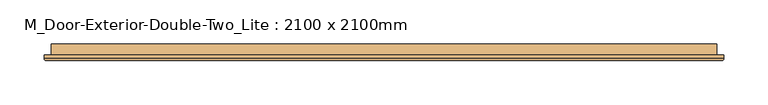
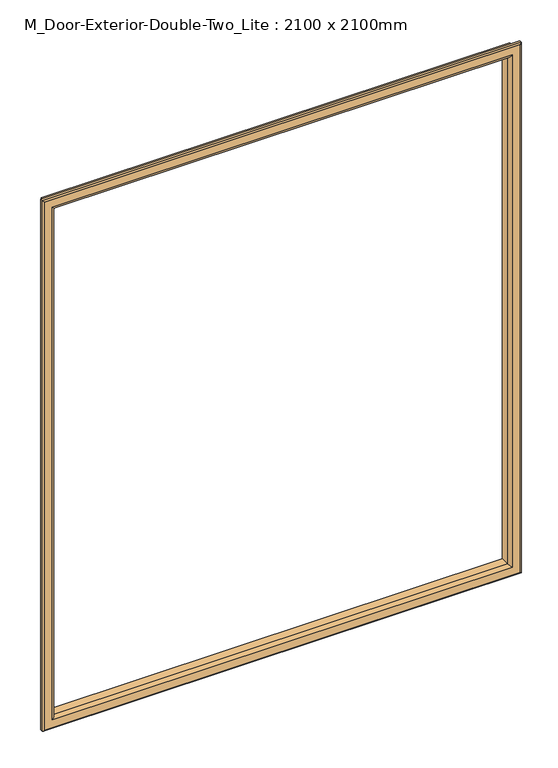
"""IFC4 building model written with IfcOpenShell, lengths in millimetres: door geometry, M_Door-Exterior-Double-Two_Lite : 2100 x 2100mm."""

from ifc_helpers import new_model, si_unit, frame, origin, place, context, project, spatial, ellipse_curve, source, transform, mapped, element, save
from ifc_brep_helpers import plane_surface, cylinder_surface, advanced_brep


def m_door_exterior_double_two_lite_2100_x_2100mm_02d4f706(model_context):
    return source(origin(), model_context, "Body", "AdvancedBrep", [
        advanced_brep(
        [(-900.0, 11.35, 1100.0), (-900.0, -1.15, 1100.0), (-900.0, -1.15, 1980.0), (-900.0, 11.35, 1980.0), (-888.0, -2.15, 1112.0), (-888.0, 11.35, 1112.0), (-888.0, 11.35, 1968.0), (-888.0, -2.15, 1968.0), (-893.0, -7.15, 1107.0), (-893.0, -7.15, 1973.0), (-908.0, -5.15, 1092.0), (-906.0, -7.15, 1094.0), (-906.0, -7.15, 1986.0), (-908.0, -5.15, 1988.0), (-908.0, -1.15, 1092.0), (-908.0, -1.15, 1988.0), (-150.0, -1.15, 1980.0), (-150.0, 11.35, 1980.0), (-162.0, 11.35, 1968.0), (-162.0, -2.15, 1968.0), (-157.0, -7.15, 1973.0), (-144.0, -7.15, 1986.0), (-142.0, -5.15, 1988.0), (-142.0, -1.15, 1988.0), (-150.0, -1.15, 1100.0), (-150.0, 11.35, 1100.0), (-162.0, 11.35, 1112.0), (-162.0, -2.15, 1112.0), (-157.0, -7.15, 1107.0), (-144.0, -7.15, 1094.0), (-142.0, -5.15, 1092.0), (-142.0, -1.15, 1092.0)],
        [
            (0, 1),
            (1, 2),
            (2, 3),
            (3, 0),
            (4, 5),
            (5, 6),
            (6, 7),
            (7, 4),
            (8, 4, ellipse_curve(frame((-893.0, -2.15, 1107.0), z_axis=(-0.7071067811865475, 0.0, 0.7071067811865475), x_axis=(-0.7071067811865474, 0.0, -0.7071067811865476)), 7.0710678, 5.0)),
            (7, 9, ellipse_curve(frame((-893.0, -2.15, 1973.0), z_axis=(-0.7071067811865475, 0.0, -0.7071067811865475), x_axis=(0.7071067811865474, 0.0, -0.7071067811865476)), 7.0710678, 5.0)),
            (9, 8),
            (10, 11, ellipse_curve(frame((-906.0, -5.15, 1094.0), z_axis=(-0.7071067811865475, 0.0, 0.7071067811865475), x_axis=(-0.7071067811865474, 0.0, -0.7071067811865476)), 2.8284271, 2.0)),
            (11, 12),
            (12, 13, ellipse_curve(frame((-906.0, -5.15, 1986.0), z_axis=(-0.7071067811865475, 0.0, -0.7071067811865475), x_axis=(0.7071067811865474, 0.0, -0.7071067811865476)), 2.8284271, 2.0)),
            (13, 10),
            (14, 10),
            (13, 15),
            (15, 14),
            (2, 16),
            (16, 17),
            (17, 3),
            (6, 18),
            (18, 19),
            (19, 7),
            (19, 20, ellipse_curve(frame((-157.0, -2.15, 1973.0), z_axis=(-0.7071067811865475, 0.0, 0.7071067811865475), x_axis=(-0.7071067811865476, 0.0, -0.7071067811865474)), 7.0710678, 5.0)),
            (20, 9),
            (12, 21),
            (21, 22, ellipse_curve(frame((-144.0, -5.15, 1986.0), z_axis=(-0.7071067811865475, 0.0, 0.7071067811865475), x_axis=(-0.7071067811865476, 0.0, -0.7071067811865474)), 2.8284271, 2.0)),
            (22, 13),
            (22, 23),
            (23, 15),
            (16, 24),
            (24, 25),
            (25, 17),
            (18, 26),
            (26, 27),
            (27, 19),
            (27, 28, ellipse_curve(frame((-157.0, -2.15, 1107.0), z_axis=(0.7071067811865475, 0.0, 0.7071067811865475), x_axis=(-0.7071067811865474, 0.0, 0.7071067811865476)), 7.0710678, 5.0)),
            (28, 20),
            (21, 29),
            (29, 30, ellipse_curve(frame((-144.0, -5.15, 1094.0), z_axis=(0.7071067811865475, 0.0, 0.7071067811865475), x_axis=(-0.7071067811865474, 0.0, 0.7071067811865476)), 2.8284271, 2.0)),
            (30, 22),
            (30, 31),
            (31, 23),
            (31, 14),
            (1, 24),
            (0, 25),
            (5, 26),
            (4, 27),
            (8, 28),
            (11, 29),
            (10, 30),
        ],
        [
            plane_surface(frame((-900.0, -1.15, 1100.0), z_axis=(-1.0, 0.0, 0.0), x_axis=(0.0, 0.0, 1.0))),
            plane_surface(frame((-888.0, 11.35, 1112.0), z_axis=(1.0, 0.0, 0.0), x_axis=(0.0, 0.0, 1.0))),
            cylinder_surface(frame((-893.0, -2.15, 1100.0), z_axis=(0.0, 0.0, -1.0), x_axis=(-1.0, 0.0, 0.0)), 5.0),
            cylinder_surface(frame((-906.0, -5.15, 1100.0), z_axis=(0.0, 0.0, -1.0), x_axis=(-1.0, 0.0, 0.0)), 2.0),
            plane_surface(frame((-908.0, -5.15, 1092.0), z_axis=(-1.0, 0.0, 0.0), x_axis=(0.0, 0.0, 1.0))),
            plane_surface(frame((-900.0, -1.15, 1980.0), z_axis=(0.0, 0.0, 1.0), x_axis=(1.0, 0.0, 0.0))),
            plane_surface(frame((-888.0, 11.35, 1968.0), z_axis=(0.0, 0.0, -1.0), x_axis=(1.0, 0.0, 0.0))),
            cylinder_surface(frame((-900.0, -2.15, 1973.0), z_axis=(-1.0, 0.0, 0.0), x_axis=(0.0, 0.0, 1.0)), 5.0),
            cylinder_surface(frame((-900.0, -5.15, 1986.0), z_axis=(-1.0, 0.0, 0.0), x_axis=(0.0, 0.0, 1.0)), 2.0),
            plane_surface(frame((-908.0, -5.15, 1988.0), z_axis=(0.0, 0.0, 1.0), x_axis=(1.0, 0.0, 0.0))),
            plane_surface(frame((-150.0, -1.15, 1980.0), z_axis=(1.0, 0.0, 0.0), x_axis=(0.0, 0.0, -1.0))),
            plane_surface(frame((-162.0, 11.35, 1968.0), z_axis=(-1.0, 0.0, 0.0), x_axis=(0.0, 0.0, -1.0))),
            cylinder_surface(frame((-157.0, -2.15, 1980.0), z_axis=(0.0, 0.0, 1.0), x_axis=(1.0, 0.0, 0.0)), 5.0),
            cylinder_surface(frame((-144.0, -5.15, 1980.0), z_axis=(0.0, 0.0, 1.0), x_axis=(1.0, 0.0, 0.0)), 2.0),
            plane_surface(frame((-142.0, -5.15, 1988.0), z_axis=(1.0, 0.0, 0.0), x_axis=(0.0, 0.0, -1.0))),
            plane_surface(frame((-142.0, -1.15, 1092.0), z_axis=(0.0, 1.0, 0.0), x_axis=(-1.0, 0.0, 0.0))),
            plane_surface(frame((-150.0, -1.15, 1100.0), z_axis=(0.0, 0.0, -1.0), x_axis=(-1.0, 0.0, 0.0))),
            plane_surface(frame((-150.0, 11.35, 1100.0), z_axis=(0.0, 1.0, 0.0), x_axis=(-1.0, 0.0, 0.0))),
            plane_surface(frame((-162.0, 11.35, 1112.0), z_axis=(0.0, 0.0, 1.0), x_axis=(-1.0, 0.0, 0.0))),
            cylinder_surface(frame((-150.0, -2.15, 1107.0), z_axis=(1.0, 0.0, 0.0), x_axis=(0.0, 0.0, -1.0)), 5.0),
            plane_surface(frame((-157.0, -7.15, 1107.0), z_axis=(0.0, -1.0, 0.0), x_axis=(-1.0, 0.0, 0.0))),
            cylinder_surface(frame((-150.0, -5.15, 1094.0), z_axis=(1.0, 0.0, 0.0), x_axis=(0.0, 0.0, -1.0)), 2.0),
            plane_surface(frame((-142.0, -5.15, 1092.0), z_axis=(0.0, 0.0, -1.0), x_axis=(-1.0, 0.0, 0.0))),
        ],
        [
            (0, [[1, 2, 3, 4]]),
            (1, [[5, 6, 7, 8]]),
            (2, [[9, -8, 10, 11]]),
            (3, [[12, 13, 14, 15]]),
            (4, [[16, -15, 17, 18]]),
            (5, [[-3, 19, 20, 21]]),
            (6, [[-7, 22, 23, 24]]),
            (7, [[-10, -24, 25, 26]]),
            (8, [[-14, 27, 28, 29]]),
            (9, [[-17, -29, 30, 31]]),
            (10, [[-20, 32, 33, 34]]),
            (11, [[-23, 35, 36, 37]]),
            (12, [[-25, -37, 38, 39]]),
            (13, [[-28, 40, 41, 42]]),
            (14, [[-30, -42, 43, 44]]),
            (15, [[-31, -44, 45, -18], [46, -32, -19, -2]]),
            (16, [[-33, -46, -1, 47]]),
            (17, [[-21, -34, -47, -4], [48, -35, -22, -6]]),
            (18, [[-36, -48, -5, 49]]),
            (19, [[-38, -49, -9, 50]]),
            (20, [[51, -40, -27, -13], [-26, -39, -50, -11]]),
            (21, [[-41, -51, -12, 52]]),
            (22, [[-43, -52, -16, -45]]),
        ],
    ),
    ])


if __name__ == "__main__":
    model = new_model("IFC4")
    model_context = context("Model", 3, world=origin())
    ifc_project = project(units=[si_unit("LENGTHUNIT", "METRE", prefix="MILLI")], contexts=[model_context])
    site = spatial("IfcSite", under=ifc_project)
    building = spatial("IfcBuilding", under=site)
    placement = place(None, origin())
    m_door_exterior_double_two_lite_2100_x_2100mm_shape = m_door_exterior_double_two_lite_2100_x_2100mm_02d4f706(model_context)
    element("IfcDoor", 1, ObjectType="M_Door-Exterior-Double-Two_Lite : 2100 x 2100mm", at=placement, inside=building, context=model_context, shape_type="MappedRepresentation", body=[
        mapped(m_door_exterior_double_two_lite_2100_x_2100mm_shape, transform((0.0, 0.0, 0.0), x_axis=(1.0, 0.0, 0.0), y_axis=(0.0, 1.0, 0.0), z_axis=(0.0, 0.0, 1.0))),
    ])
    save(model, "model.ifc")

# Revit data of these elements
# Type "M_Door-Exterior-Double-Two_Lite : 2100 x 2100mm"
#   Type Mark = "46"
#   Assembly Code = "B2030100"
#   Analytic Construction = "Metal frame, double glass door"
#   Top Rail = 120 mm
#   Threshold Length [instance default] = 2200 mm
#   Threshold Offset [instance default] = 15 mm
#   Thickness = 45 mm
#   Thermal Resistance (R) = 0.242926 (m²·K)/W
#   Swing Angle [instance default] = 90.00°
#   Strike Height = 1000 mm
#   Stiles = 150 mm
#   SinglePanelWidth = 1050 mm
#   Rough Width [instance default] = 2200 mm
#   Rough Height [instance default] = 2200 mm
#   MFOpeningHeight [instance default] = 100 mm
#   MFOpeningWidth [instance default] = 100 mm
#   Lock Rail = 200 mm
#   Inset Calculate [instance default] = 105 mm
#   Masonry Inset [instance default] = 25 mm
#   Height = 2100 mm
#   Width = 2100 mm
#   Heat Transfer Coefficient (U) = 4.11674 W/(m²·K)
#   Glass Thickness = 20 mm
#   Masonry Frame Depth = 150 mm
#   Bottom Rail = 250 mm
#   Threshold [instance default] = yes
#   Masonry Frame [instance default] = yes
#   Function = 1
#   Dry Wall Frame [instance default] = no
#   Threshold Material = Cherry
#   Panic Bar Material = Metal - Stainless Steel
#   Panel Material = Metal - Painted - Grey
#   Glass Stop Material = Metal - Painted - Grey
#   Frame Material = Metal - Painted - Grey
#   Exterior Pull Material = Metal - Stainless Steel
#   Visual Light Transmittance = 0
#   Solar Heat Gain Coefficient = 0
#   Wall Closure = (empty or 0)
# Element 1 (IfcDoor, "M_Door-Exterior-Double-Two_Lite : 2100 x 2100mm")
#   Materials on its faces: "Metal - Painted - Grey", "Metal - Stainless Steel", "Glass", "Cherry"
# Materials
#   "Cherry": class "Wood", colour RGB 226 177 128, transparency 0, Description = "Prunus Serotina", Cost = 0
#   "Metal - Stainless Steel": class "Metal", colour RGB 247 247 247, transparency 0
#   "Metal - Painted - Grey": class "Paint", colour RGB 104 104 104, transparency 0, Cost = 0
#   "Glass": class "Glass", colour RGB 0 128 192, transparency 0.9, Description = "Soda Lime Glass", Cost = 0
